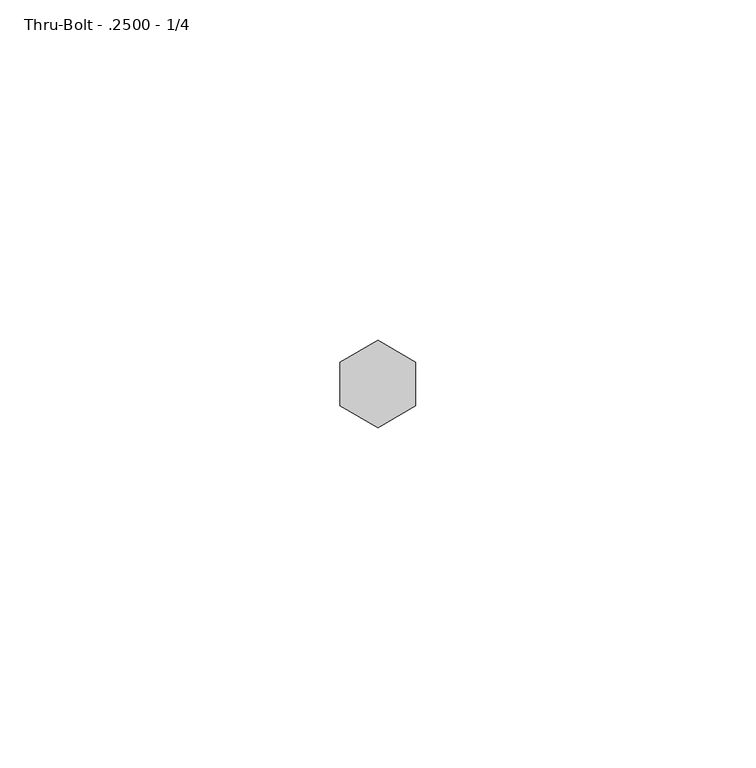
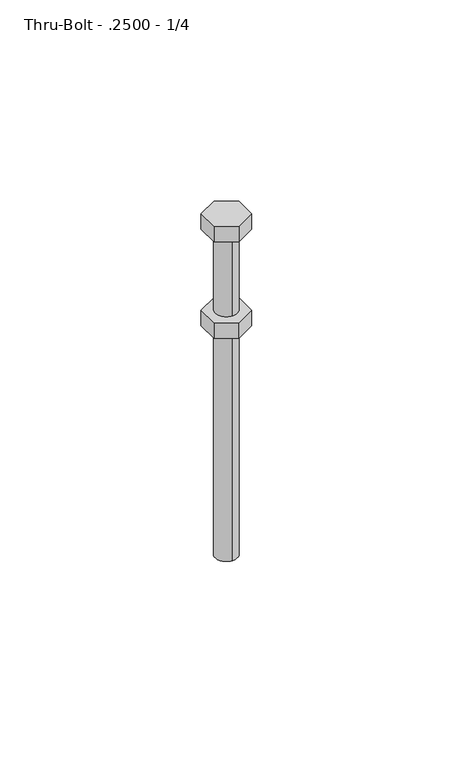
"""IFC4 building model written with IfcOpenShell, lengths in millimetres: fastener geometry, 060523 - W_P_C - Fastenings - Generic : Thru-Bolt - .2500 - 1/4."""

import ifcopenshell
import ifcopenshell.guid

model = None  # the IFC model being written
_history = None  # IfcOwnerHistory: only IFC2X3 demands one
_inside = {}  # id of a spatial element -> (the spatial element, [elements in it])
_under = {}  # id of a project, library or spatial element -> (it, [spatial elements below it])
_declared = {}  # id of a project -> (the project, [libraries it declares])
_typed = {}  # id of a type object -> (the type object, [elements of that type])
_made_of = {}  # id of a material, layer set ... -> (it, [elements and type objects made of it])


def new_model(schema):
    """Start an empty IFC model of exactly this schema.

    Asked for "IFC4X3", IfcOpenShell would pick the latest addendum, in which some entities
    have other attributes; the version numbers below select the first issue.
    IFC2X3 requires an IfcOwnerHistory on every rooted entity: one is made here for all.
    """
    global model, _history
    if schema == "IFC4X3":
        model = ifcopenshell.file(schema_version=(4, 3, 0, 0))
    else:
        model = ifcopenshell.file(schema=schema)
    _inside.clear()
    _under.clear()
    _declared.clear()
    _typed.clear()
    _made_of.clear()
    _history = None
    if model.schema == "IFC2X3":
        org = make("IfcOrganization", Name="unknown")
        user = make(
            "IfcPersonAndOrganization",
            ThePerson=make("IfcPerson", FamilyName="unknown"),
            TheOrganization=org,
        )
        app = make(
            "IfcApplication",
            ApplicationDeveloper=org,
            Version="unknown",
            ApplicationFullName="unknown",
            ApplicationIdentifier="unknown",
        )
        _history = make(
            "IfcOwnerHistory",
            OwningUser=user,
            OwningApplication=app,
            ChangeAction="ADDED",
            CreationDate=0,
        )
    return model


def make(cls, **values):
    """One entity of the class cls with the attributes given. An attribute that is None is left unset."""
    return model.create_entity(
        cls, **{name: value for name, value in values.items() if value is not None}
    )


def rooted(cls, **values):
    """An entity with a GlobalId (a new one), such as an element, a storey or a relation."""
    return make(cls, GlobalId=ifcopenshell.guid.new(), OwnerHistory=_history, **values)


def si_unit(unit_type, name, prefix=None):
    """IfcSIUnit, for example si_unit("LENGTHUNIT", "METRE", prefix="MILLI")."""
    return make("IfcSIUnit", UnitType=unit_type, Prefix=prefix, Name=name)


def assignment(units):
    """IfcUnitAssignment: the units of a project."""
    return None if units is None else make("IfcUnitAssignment", Units=units)


def point(xyz):
    """IfcCartesianPoint."""
    return None if xyz is None else make("IfcCartesianPoint", Coordinates=xyz)


def direction(xyz):
    """IfcDirection."""
    return None if xyz is None else make("IfcDirection", DirectionRatios=xyz)


def frame(location, z_axis=None, x_axis=None):
    """IfcAxis2Placement3D, a coordinate frame: its origin and axes. An axis left out is left unset."""
    return make(
        "IfcAxis2Placement3D",
        Location=point(location),
        Axis=direction(z_axis),
        RefDirection=direction(x_axis),
    )


def frame_2d(location, x_axis=None):
    """IfcAxis2Placement2D, a coordinate frame in the plane: its origin and x axis."""
    return make(
        "IfcAxis2Placement2D", Location=point(location), RefDirection=direction(x_axis)
    )


def origin():
    """The frame at (0, 0, 0) with its axes left unset."""
    return frame((0.0, 0.0, 0.0))


def origin_with_axes():
    """The frame at (0, 0, 0) with the z axis (0, 0, 1) and the x axis (1, 0, 0) written out."""
    return frame((0.0, 0.0, 0.0), z_axis=(0.0, 0.0, 1.0), x_axis=(1.0, 0.0, 0.0))


def origin_2d():
    """The frame at (0, 0) in the plane with its x axis left unset."""
    return frame_2d((0.0, 0.0))


def place(relative_to, where):
    """IfcLocalPlacement: puts the frame where relative to a parent placement (None: the world)."""
    return make(
        "IfcLocalPlacement", PlacementRelTo=relative_to, RelativePlacement=where
    )


def context(
    kind, dimensions, precision=None, world=None, true_north=None, identifier=None
):
    """IfcGeometricRepresentationContext, for example the 3D "Model" context."""
    return make(
        "IfcGeometricRepresentationContext",
        ContextIdentifier=identifier,
        ContextType=kind,
        CoordinateSpaceDimension=dimensions,
        Precision=precision,
        WorldCoordinateSystem=world,
        TrueNorth=true_north,
    )


def project(units=None, contexts=None):
    """IfcProject with its units and contexts."""
    return rooted(
        "IfcProject",
        Name="project",
        RepresentationContexts=contexts,
        UnitsInContext=assignment(units),
    )


def spatial(cls, under=None, at=None, **own):
    """A site, building, storey or space (cls), placed at a placement, below another one or the project."""
    s = rooted(cls, ObjectPlacement=at, **own)
    if under is not None:
        _under.setdefault(under.id(), (under, []))[1].append(s)
    return s


def polyline(points):
    """IfcPolyline through the points."""
    return make("IfcPolyline", Points=[point(p) for p in points])


def circle_curve(where, radius):
    """IfcCircle in the frame where."""
    return make("IfcCircle", Position=where, Radius=radius)


def trimmed(basis, trim1, trim2, sense, master):
    """IfcTrimmedCurve: the piece of a basis curve between two trims."""
    return make(
        "IfcTrimmedCurve",
        BasisCurve=basis,
        Trim1=trim1,
        Trim2=trim2,
        SenseAgreement=sense,
        MasterRepresentation=master,
    )


def segment(curve, same_sense, transition):
    """IfcCompositeCurveSegment."""
    return make(
        "IfcCompositeCurveSegment",
        Transition=transition,
        SameSense=same_sense,
        ParentCurve=curve,
    )


def composite_curve(segments, self_intersect=None):
    """IfcCompositeCurve: segments joined end to end."""
    return make("IfcCompositeCurve", Segments=segments, SelfIntersect=self_intersect)


def outline(outer, holes=None, kind="AREA"):
    """IfcArbitraryClosedProfileDef: a profile drawn as a closed curve; with holes, ...WithVoids."""
    if holes is None:
        return make("IfcArbitraryClosedProfileDef", ProfileType=kind, OuterCurve=outer)
    return make(
        "IfcArbitraryProfileDefWithVoids",
        ProfileType=kind,
        OuterCurve=outer,
        InnerCurves=holes,
    )


def extrude(swept, where, along, depth):
    """IfcExtrudedAreaSolid: the profile swept, set in the frame where, extruded along a direction by depth."""
    return make(
        "IfcExtrudedAreaSolid",
        SweptArea=swept,
        Position=where,
        ExtrudedDirection=direction(along),
        Depth=depth,
    )


def shape(context_of_items, identifier, shape_type, items):
    """IfcShapeRepresentation: the items that make up one representation, for example the "Body"."""
    return make(
        "IfcShapeRepresentation",
        ContextOfItems=context_of_items,
        RepresentationIdentifier=identifier,
        RepresentationType=shape_type,
        Items=items,
    )


def source(mapping_origin, context_of_items, identifier, shape_type, items):
    """IfcRepresentationMap: a shape defined once, which mapped items show again and again."""
    return make(
        "IfcRepresentationMap",
        MappingOrigin=mapping_origin,
        MappedRepresentation=shape(context_of_items, identifier, shape_type, items),
    )


def transform(
    local_origin,
    x_axis=None,
    y_axis=None,
    z_axis=None,
    scale=None,
    scale2=None,
    scale3=None,
    uniform=True,
):
    """IfcCartesianTransformationOperator3D, or its non-uniform kind. x_axis, y_axis, z_axis: its Axis1, 2, 3."""
    if uniform:
        return make(
            "IfcCartesianTransformationOperator3D",
            Axis1=direction(x_axis),
            Axis2=direction(y_axis),
            LocalOrigin=point(local_origin),
            Scale=scale,
            Axis3=direction(z_axis),
        )
    return make(
        "IfcCartesianTransformationOperator3DnonUniform",
        Axis1=direction(x_axis),
        Axis2=direction(y_axis),
        LocalOrigin=point(local_origin),
        Scale=scale,
        Axis3=direction(z_axis),
        Scale2=scale2,
        Scale3=scale3,
    )


def mapped(mapping_source, mapping_target):
    """IfcMappedItem: shows the shape of a source again, moved by a transform."""
    return make(
        "IfcMappedItem", MappingSource=mapping_source, MappingTarget=mapping_target
    )


def made_of(thing, what):
    """Note that an element or type object is made of a material, layer set ...; save() writes the relation."""
    if what is not None:
        _made_of.setdefault(what.id(), (what, []))[1].append(thing)
    return thing


def element(
    cls,
    number,
    at=None,
    inside=None,
    cuts=None,
    type_object=None,
    material=None,
    context=None,
    identifier="Body",
    shape_type=None,
    held_by="IfcProductDefinitionShape",
    body=None,
    shapes=None,
    **own,
):
    """One element of the class cls, such as IfcWall. Its Tag is "e" and its number.

    at: its placement. inside: the storey or other place that contains it. cuts: it is an
    opening in that element (IfcRelVoidsElement). A single representation is given by context,
    identifier, shape_type and body (its items); several are given by shapes. held_by: the class
    of the entity that holds the representations. save() writes the other relations.
    """
    e = rooted(cls, Tag="e%d" % number, ObjectPlacement=at, **own)
    if body is not None:
        shapes = [shape(context, identifier, shape_type, body)]
    if shapes is not None:
        e.Representation = make(held_by, Representations=shapes)
    if inside is not None:
        _inside.setdefault(inside.id(), (inside, []))[1].append(e)
    if cuts is not None:
        rooted(
            "IfcRelVoidsElement", RelatingBuildingElement=cuts, RelatedOpeningElement=e
        )
    if type_object is not None:
        _typed.setdefault(type_object.id(), (type_object, []))[1].append(e)
    return made_of(e, material)


def aggregate(whole, parts):
    """IfcRelAggregates: a whole, such as a stair, and the parts it consists of."""
    return rooted("IfcRelAggregates", RelatingObject=whole, RelatedObjects=parts)


def save(model, path):
    """Write the relations noted so far, then the file.

    IfcRelAggregates (storeys below a building ...), IfcRelContainedInSpatialStructure (elements
    in a storey), IfcRelDefinesByType, IfcRelAssociatesMaterial and IfcRelDeclares: one each for
    every whole, place, type object, material and project.
    """
    for whole, parts in _under.values():
        aggregate(whole, parts)
    for where, things in _inside.values():
        rooted(
            "IfcRelContainedInSpatialStructure",
            RelatedElements=things,
            RelatingStructure=where,
        )
    for kind, things in _typed.values():
        rooted("IfcRelDefinesByType", RelatedObjects=things, RelatingType=kind)
    for what, things in _made_of.values():
        rooted("IfcRelAssociatesMaterial", RelatedObjects=things, RelatingMaterial=what)
    for by, libraries in _declared.values():
        rooted("IfcRelDeclares", RelatingContext=by, RelatedDefinitions=libraries)
    model.write(path)


def thru_bolt_2500_1_4_4b19fb5d(model_context):
    return source(origin(), model_context, "Body", "SweptSolid", [
        extrude(outline(polyline([(-5.55625, -3.2079024), (-5.55625, 3.2079024), (0.0, 6.4158049), (5.55625, 3.2079024), (5.55625, -3.2079024), (0.0, -6.4158049), (-5.55625, -3.2079024)])), frame((0.0, 0.0, -30.1625), z_axis=(0.0, 0.0, 1.0), x_axis=(1.0, 0.0, 0.0)), (0.0, 0.0, 1.0), 4.7625),
        extrude(outline(polyline([(-5.55625, 3.2079024), (0.0, 6.4158049), (5.55625, 3.2079024), (5.55625, -3.2079024), (0.0, -6.4158049), (-5.55625, -3.2079024), (-5.55625, 3.2079024)])), origin_with_axes(), (0.0, 0.0, 1.0), 4.7625),
        extrude(outline(composite_curve([segment(trimmed(circle_curve(origin_2d(), 3.302), [point((0.0, -3.302))], [point((0.0, 3.302))], False, "CARTESIAN"), True, "CONTINUOUS"), segment(trimmed(circle_curve(origin_2d(), 3.302), [point((0.0, 3.302))], [point((0.0, -3.302))], False, "CARTESIAN"), True, "CONTINUOUS")], self_intersect=False)), frame((0.0, 0.0, -101.6), z_axis=(0.0, 0.0, 1.0), x_axis=(1.0, 0.0, 0.0)), (0.0, 0.0, 1.0), 101.6),
    ])


if __name__ == "__main__":
    model = new_model("IFC4")
    model_context = context("Model", 3, world=origin())
    ifc_project = project(units=[si_unit("LENGTHUNIT", "METRE", prefix="MILLI")], contexts=[model_context])
    site = spatial("IfcSite", under=ifc_project)
    building = spatial("IfcBuilding", under=site)
    placement = place(None, origin())
    thru_bolt_2500_1_4_shape = thru_bolt_2500_1_4_4b19fb5d(model_context)
    element("IfcFastener", 1, ObjectType="060523 - W_P_C - Fastenings - Generic : Thru-Bolt - .2500 - 1/4", at=placement, inside=building, context=model_context, shape_type="MappedRepresentation", body=[
        mapped(thru_bolt_2500_1_4_shape, transform((0.0, 0.0, 0.0), x_axis=(1.0, 0.0, 0.0), y_axis=(0.0, 1.0, 0.0), z_axis=(0.0, 0.0, 1.0))),
    ])
    save(model, "model.ifc")

# Revit data of these elements
# Type "060523 - W_P_C - Fastenings - Generic : Thru-Bolt - .2500 - 1/4"
#   Washer_Thickness = 0' - 0 1/16"
#   Washer Radius = 0' - 0.3175"
#   Washer Offset - Head = 0' - 0"
#   Washer Offset = 0' - 0"
#   Thickness_of_Substrate [instance default] = 0' - 1"
#   Side = 0' - 0.25293"
#   Radius = 0' - 0.13"
#   Length [instance default] = 0' - 4"
#   Head Size = 0' - 0 7/16"
#   Head Radius = 0' - 0 7/32"
#   Head Height = 0' - 0 3/16"
#   Double Diameter = 0' - 0.52"
#   Diameter = 0' - 0.26"
#   Default Elevation = 4' - 0"
#   Washer_Nut_Visibility = no
#   Washer_Head_Visibility = no
#   Round_Head_Visibility = no
#   Point Visibility = no
#   Nut_Visibility = yes
#   Hex_Head_Visiblilty = yes
#   Washer Material = none
#   Bolt Material (Size) = AT SILL - FASTENER AT 24" O.C.
# Element 1 (IfcFastener, "060523 - W_P_C - Fastenings - Generic : Thru-Bolt - .2500 - 1/4")
#   Materials on its faces: "AT SILL - FASTENER AT 24\" O.C."
# Materials
#   "AT SILL - FASTENER AT 24\" O.C.": class "Generic", colour RGB 120 120 120, transparency 0, Cost = 0
